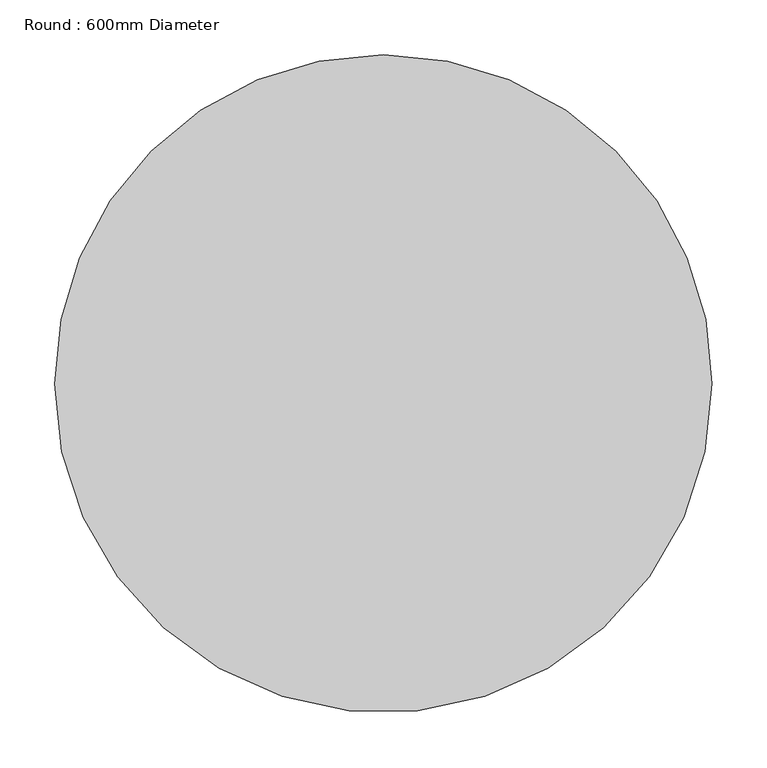
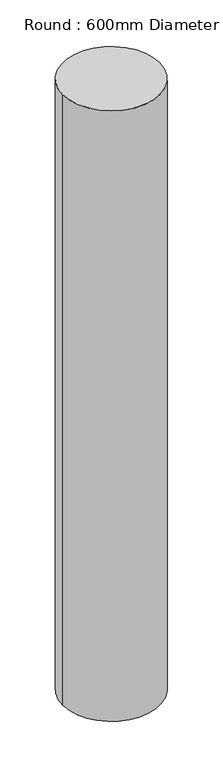
"""IFC4 building model written with IfcOpenShell, lengths in millimetres: column geometry, Round : 600mm Diameter."""

from ifc_helpers import new_model, si_unit, point, frame, origin, origin_2d, place, context, project, spatial, circle_curve, trimmed, segment, composite_curve, outline, extrude, source, transform, mapped, element, save


def round_600mm_diameter_b114da78(model_context):
    return source(origin(), model_context, "Body", "SweptSolid", [
        extrude(outline(composite_curve([segment(trimmed(circle_curve(origin_2d(), 300.0), [point((300.0, 0.0))], [point((-300.0, 0.0))], False, "CARTESIAN"), True, "CONTINUOUS"), segment(trimmed(circle_curve(origin_2d(), 300.0), [point((-300.0, 0.0))], [point((0.0, 300.0))], False, "CARTESIAN"), True, "CONTINUOUS"), segment(trimmed(circle_curve(origin_2d(), 300.0), [point((0.0, 300.0))], [point((300.0, 0.0))], False, "CARTESIAN"), True, "CONTINUOUS")], self_intersect=False)), frame((0.0, 0.0, 134670.0), z_axis=(0.0, 0.0, 1.0), x_axis=(1.0, 0.0, 0.0)), (0.0, 0.0, 1.0), 4000.0),
    ])


if __name__ == "__main__":
    model = new_model("IFC4")
    model_context = context("Model", 3, world=origin())
    ifc_project = project(units=[si_unit("LENGTHUNIT", "METRE", prefix="MILLI")], contexts=[model_context])
    site = spatial("IfcSite", under=ifc_project)
    building = spatial("IfcBuilding", under=site)
    placement = place(None, origin())
    round_600mm_diameter_shape = round_600mm_diameter_b114da78(model_context)
    element("IfcColumn", 1, ObjectType="Round : 600mm Diameter", at=placement, inside=building, context=model_context, shape_type="MappedRepresentation", body=[
        mapped(round_600mm_diameter_shape, transform((0.0, 0.0, 0.0), x_axis=(1.0, 0.0, 0.0), y_axis=(0.0, 1.0, 0.0), z_axis=(0.0, 0.0, 1.0))),
    ])
    save(model, "model.ifc")

# Revit data of these elements
# Type "Round : 600mm Diameter"
#   Keynote = "G"
#   Diameter = 600.00 mm
#   Offset Base = 0.00 mm
#   Offset Top = 0.00 mm
#   built-in parameter 1002110 = 8421504
#   built-in parameter 1002106 = element 3
#   Material = Concrete - Cast In Situ
# Element 1 (IfcColumn, "Round : 600mm Diameter")
#   Materials on its faces: "Concrete - Cast In Situ"
# Materials
#   "Concrete - Cast In Situ": class "Unassigned", colour RGB 255 255 255, transparency 0, Keynote = "E10/132", Cost = 0
